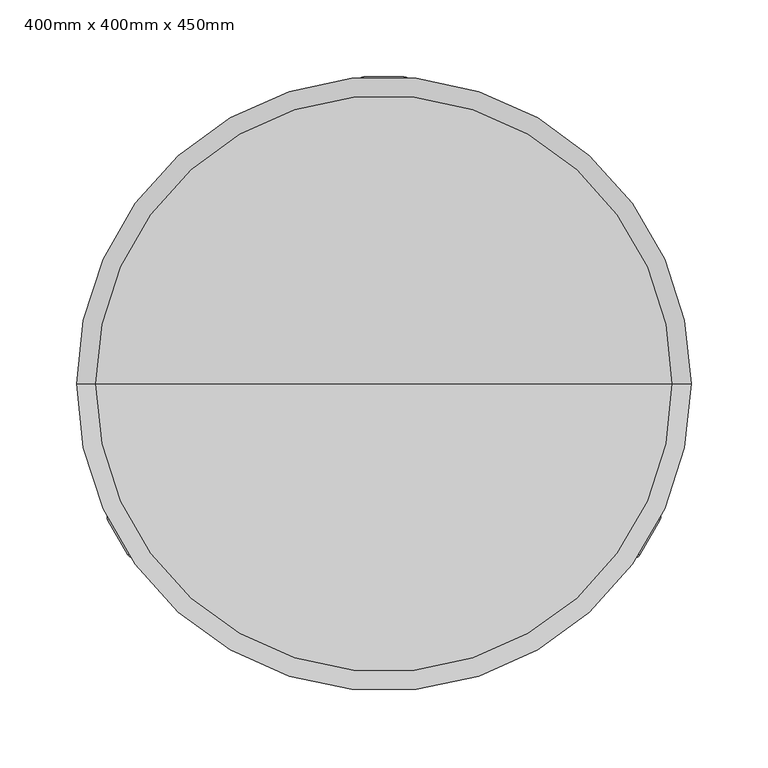
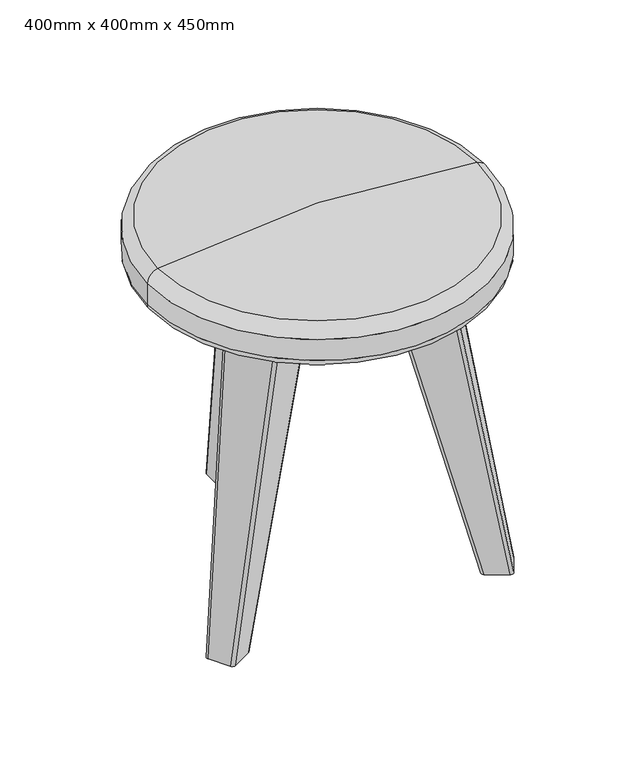
"""IFC4 building model written with IfcOpenShell, lengths in millimetres: furniture geometry, Seating-Casual-James_Burleigh-Shug : 400mm x 400mm x 450mm."""

from ifc_helpers import new_model, si_unit, point, frame, origin, place, context, project, spatial, circle_curve, ellipse_curve, trimmed, source, transform, mapped, element, save
from ifc_brep_helpers import plane_surface, cylinder_surface, revolved_surface, extruded_surface, advanced_brep


def furniture_400mm_x_400mm_x_450mm_e073d23b(model_context):
    return source(origin(), model_context, "Body", "AdvancedBrep", [
        advanced_brep(
        [(-100.6813787, -91.6147367, 384.0), (-95.2172771, -93.0788383, 384.0), (-44.9878037, -64.0788383, 384.0), (-43.5237021, -58.6147367, 384.0), (-72.5237021, -8.3852633, 384.0), (-77.9878037, -6.9211617, 384.0), (-128.2172771, -35.9211617, 384.0), (-129.6813787, -41.3852633, 384.0), (-166.7050808, -111.2583302, 0.0), (-179.7050808, -88.7416698, 0.0), (-178.2409791, -83.2775681, 0.0), (-155.7243186, -70.2775681, 0.0), (-150.260217, -71.7416698, 0.0), (-137.260217, -94.2583302, 0.0), (-138.7243186, -99.7224319, 0.0), (-161.2409791, -112.7224319, 0.0)],
        [
            (0, 1, circle_curve(frame((-97.2172771, -89.6147367, 384.0), z_axis=(0.0, 0.0, 1.0), x_axis=(-0.49999999999999306, 0.8660254037844427, 0.0)), 4.0)),
            (1, 2),
            (2, 3, circle_curve(frame((-46.9878037, -60.6147367, 384.0), z_axis=(0.0, 0.0, 1.0), x_axis=(-0.49999999999999306, 0.8660254037844427, 0.0)), 4.0)),
            (3, 4),
            (4, 5, circle_curve(frame((-75.9878037, -10.3852633, 384.0), z_axis=(0.0, 0.0, 1.0), x_axis=(-0.49999999999999306, 0.8660254037844427, 0.0)), 4.0)),
            (5, 6),
            (6, 7, circle_curve(frame((-126.2172771, -39.3852633, 384.0), z_axis=(0.0, 0.0, 1.0), x_axis=(-0.49999999999999306, 0.8660254037844427, 0.0)), 4.0)),
            (7, 0),
            (8, 9),
            (9, 10, circle_curve(frame((-176.2409791, -86.7416698, 0.0), z_axis=(0.0, 0.0, -1.0), x_axis=(-0.49999999999999306, 0.8660254037844427, 0.0)), 4.0)),
            (10, 11),
            (11, 12, circle_curve(frame((-153.7243186, -73.7416698, 0.0), z_axis=(0.0, 0.0, -1.0), x_axis=(-0.49999999999999306, 0.8660254037844427, 0.0)), 4.0)),
            (12, 13),
            (13, 14, circle_curve(frame((-140.7243186, -96.2583302, 0.0), z_axis=(0.0, 0.0, -1.0), x_axis=(-0.49999999999999306, 0.8660254037844427, 0.0)), 4.0)),
            (14, 15),
            (15, 8, circle_curve(frame((-163.2409791, -109.2583302, 0.0), z_axis=(0.0, 0.0, -1.0), x_axis=(-0.49999999999999306, 0.8660254037844427, 0.0)), 4.0)),
            (14, 2),
            (1, 15),
            (12, 4),
            (3, 13),
            (10, 6),
            (5, 11),
            (8, 0),
            (7, 9),
        ],
        [
            plane_surface(frame((-86.6025404, -50.0, 384.0), z_axis=(0.0, 0.0, 1.0), x_axis=(0.4999999999999859, -0.8660254037844468, 0.0))),
            plane_surface(frame((-158.4826489, -91.5, 0.0), z_axis=(0.0, 0.0, -1.0), x_axis=(0.4999999999999859, -0.8660254037844468, 0.0))),
            plane_surface(frame((-149.9826489, -106.2224319, 0.0), z_axis=(0.49956653654616645, -0.8652746230591969, -0.041630544712180834), x_axis=(0.8660254037844443, 0.4999999999999904, 0.0))),
            plane_surface(frame((-143.760217, -83.0, 0.0), z_axis=(0.8386038712126963, 0.4841681707881, -0.24964921306261928), x_axis=(-0.4999999999999904, 0.8660254037844443, 0.0))),
            plane_surface(frame((-166.9826489, -76.7775681, 0.0), z_axis=(-0.49956653654616634, 0.8652746230591967, -0.04163054471218183), x_axis=(-0.8660254037844443, -0.4999999999999904, 0.0))),
            plane_surface(frame((-173.2050808, -100.0, 0.0), z_axis=(-0.8531367483367913, -0.49255873130779587, 0.17188247394595313), x_axis=(0.4999999999999904, -0.8660254037844443, 0.0))),
            extruded_surface(trimmed(circle_curve(frame((-163.2409791, -109.2583302, 0.0), z_axis=(0.0, 0.0, 1.0), x_axis=(-0.49999999999999306, 0.8660254037844427, 0.0)), 4.0), [point((-166.7050808, -111.2583302, 0.0))], [point((-161.2409791, -112.7224319, 0.0))], True, "CARTESIAN"), (66.023702, 19.64359350000001, 384.0), 390.1294656795075),
            extruded_surface(trimmed(circle_curve(frame((-140.7243186, -96.2583302, 0.0), z_axis=(0.0, 0.0, 1.0), x_axis=(-0.49999999999999306, 0.8660254037844427, 0.0)), 4.0), [point((-138.7243186, -99.7224319, 0.0))], [point((-137.260217, -94.2583302, 0.0))], True, "CARTESIAN"), (93.7365149, 35.6435935, 384.0), 396.8790747610551),
            extruded_surface(trimmed(circle_curve(frame((-153.7243186, -73.7416698, 0.0), z_axis=(0.0, 0.0, 1.0), x_axis=(-0.49999999999999306, 0.8660254037844427, 0.0)), 4.0), [point((-150.260217, -71.7416698, 0.0))], [point((-155.7243186, -70.2775681, 0.0))], True, "CARTESIAN"), (77.7365149, 63.3564065, 384.0), 396.87907477390536),
            extruded_surface(trimmed(circle_curve(frame((-176.2409791, -86.7416698, 0.0), z_axis=(0.0, 0.0, 1.0), x_axis=(-0.49999999999999306, 0.8660254037844427, 0.0)), 4.0), [point((-178.2409791, -83.2775681, 0.0))], [point((-179.7050808, -88.7416698, 0.0))], True, "CARTESIAN"), (50.023702, 47.3564065, 384.0), 390.1294656884789),
        ],
        [
            (0, [[1, 2, 3, 4, 5, 6, 7, 8]]),
            (1, [[9, 10, 11, 12, 13, 14, 15, 16]]),
            (2, [[-15, 17, -2, 18]]),
            (3, [[-13, 19, -4, 20]]),
            (4, [[-11, 21, -6, 22]]),
            (5, [[-9, 23, -8, 24]]),
            (6, [[-16, -18, -1, -23]]),
            (7, [[-14, -20, -3, -17]]),
            (8, [[-12, -22, -5, -19]]),
            (9, [[-10, -24, -7, -21]]),
        ],
    ),
        advanced_brep(
        [(129.6813787, -41.3852633, 384.0), (128.2172771, -35.9211617, 384.0), (77.9878037, -6.9211617, 384.0), (72.5237021, -8.3852633, 384.0), (43.5237021, -58.6147367, 384.0), (44.9878037, -64.0788383, 384.0), (95.2172771, -93.0788383, 384.0), (100.6813787, -91.6147367, 384.0), (179.7050808, -88.7416698, 0.0), (166.7050808, -111.2583302, 0.0), (161.2409791, -112.7224319, 0.0), (138.7243186, -99.7224319, 0.0), (137.260217, -94.2583302, 0.0), (150.260217, -71.7416698, 0.0), (155.7243186, -70.2775681, 0.0), (178.2409791, -83.2775681, 0.0)],
        [
            (0, 1, circle_curve(frame((126.2172771, -39.3852633, 384.0), z_axis=(0.0, 0.0, 1.0000000000000002), x_axis=(-0.5000000000000088, -0.8660254037844337, 0.0)), 4.0)),
            (1, 2),
            (2, 3, circle_curve(frame((75.9878037, -10.3852633, 384.0), z_axis=(0.0, 0.0, 1.0000000000000002), x_axis=(-0.5000000000000088, -0.8660254037844337, 0.0)), 4.0)),
            (3, 4),
            (4, 5, circle_curve(frame((46.9878037, -60.6147367, 384.0), z_axis=(0.0, 0.0, 1.0000000000000002), x_axis=(-0.5000000000000088, -0.8660254037844337, 0.0)), 4.0)),
            (5, 6),
            (6, 7, circle_curve(frame((97.2172771, -89.6147367, 384.0), z_axis=(0.0, 0.0, 1.0000000000000002), x_axis=(-0.5000000000000088, -0.8660254037844337, 0.0)), 4.0)),
            (7, 0),
            (8, 9),
            (9, 10, circle_curve(frame((163.2409791, -109.2583302, 0.0), z_axis=(0.0, 0.0, -1.0000000000000002), x_axis=(-0.5000000000000088, -0.8660254037844337, 0.0)), 4.0)),
            (10, 11),
            (11, 12, circle_curve(frame((140.7243186, -96.2583302, 0.0), z_axis=(0.0, 0.0, -1.0000000000000002), x_axis=(-0.5000000000000088, -0.8660254037844337, 0.0)), 4.0)),
            (12, 13),
            (13, 14, circle_curve(frame((153.7243186, -73.7416698, 0.0), z_axis=(0.0, 0.0, -1.0000000000000002), x_axis=(-0.5000000000000088, -0.8660254037844337, 0.0)), 4.0)),
            (14, 15),
            (15, 8, circle_curve(frame((176.2409791, -86.7416698, 0.0), z_axis=(0.0, 0.0, -1.0000000000000002), x_axis=(-0.5000000000000088, -0.8660254037844337, 0.0)), 4.0)),
            (14, 2),
            (1, 15),
            (12, 4),
            (3, 13),
            (10, 6),
            (5, 11),
            (8, 0),
            (7, 9),
        ],
        [
            plane_surface(frame((86.6025404, -50.0, 384.0), z_axis=(0.0, 0.0, 1.0), x_axis=(0.5000000000000152, 0.8660254037844299, 0.0))),
            plane_surface(frame((158.4826489, -91.5, 0.0), z_axis=(0.0, 0.0, -1.0), x_axis=(0.5000000000000152, 0.8660254037844299, 0.0))),
            plane_surface(frame((166.9826489, -76.7775681, 0.0), z_axis=(0.49956653654618743, 0.8652746230591847, -0.041630544712180834), x_axis=(-0.8660254037844322, 0.5000000000000114, 0.0))),
            plane_surface(frame((143.760217, -83.0, 0.0), z_axis=(-0.8386038712126845, 0.48416817078812036, -0.24964921306261922), x_axis=(-0.5000000000000114, -0.8660254037844322, 0.0))),
            plane_surface(frame((149.9826489, -106.2224319, 0.0), z_axis=(-0.4995665365461874, -0.8652746230591846, -0.04163054471218185), x_axis=(0.8660254037844322, -0.5000000000000114, 0.0))),
            plane_surface(frame((173.2050808, -100.0, 0.0), z_axis=(0.8531367483367793, -0.4925587313078165, 0.17188247394595313), x_axis=(0.5000000000000114, 0.8660254037844322, 0.0))),
            extruded_surface(trimmed(circle_curve(frame((176.2409791, -86.7416698, 0.0), z_axis=(0.0, 0.0, 1.0000000000000002), x_axis=(-0.5000000000000088, -0.8660254037844337, 0.0)), 4.0), [point((179.7050808, -88.7416698, 0.0))], [point((178.2409791, -83.2775681, 0.0))], True, "CARTESIAN"), (-50.023702, 47.3564065, 384.0), 390.1294656884789),
            extruded_surface(trimmed(circle_curve(frame((153.7243186, -73.7416698, 0.0), z_axis=(0.0, 0.0, 1.0000000000000002), x_axis=(-0.5000000000000088, -0.8660254037844337, 0.0)), 4.0), [point((155.7243186, -70.2775681, 0.0))], [point((150.260217, -71.7416698, 0.0))], True, "CARTESIAN"), (-77.7365149, 63.3564065, 384.0), 396.87907477390536),
            extruded_surface(trimmed(circle_curve(frame((140.7243186, -96.2583302, 0.0), z_axis=(0.0, 0.0, 1.0000000000000002), x_axis=(-0.5000000000000088, -0.8660254037844337, 0.0)), 4.0), [point((137.260217, -94.2583302, 0.0))], [point((138.7243186, -99.7224319, 0.0))], True, "CARTESIAN"), (-93.7365149, 35.6435935, 384.0), 396.8790747610551),
            extruded_surface(trimmed(circle_curve(frame((163.2409791, -109.2583302, 0.0), z_axis=(0.0, 0.0, 1.0000000000000002), x_axis=(-0.5000000000000088, -0.8660254037844337, 0.0)), 4.0), [point((161.2409791, -112.7224319, 0.0))], [point((166.7050808, -111.2583302, 0.0))], True, "CARTESIAN"), (-66.023702, 19.64359350000001, 384.0), 390.1294656795075),
        ],
        [
            (0, [[1, 2, 3, 4, 5, 6, 7, 8]]),
            (1, [[9, 10, 11, 12, 13, 14, 15, 16]]),
            (2, [[-15, 17, -2, 18]]),
            (3, [[-13, 19, -4, 20]]),
            (4, [[-11, 21, -6, 22]]),
            (5, [[-9, 23, -8, 24]]),
            (6, [[-16, -18, -1, -23]]),
            (7, [[-14, -20, -3, -17]]),
            (8, [[-12, -22, -5, -19]]),
            (9, [[-10, -24, -7, -21]]),
        ],
    ),
        advanced_brep(
        [(-29.0, 133.0, 384.0), (-33.0, 129.0, 384.0), (-33.0, 71.0, 384.0), (-29.0, 67.0, 384.0), (29.0, 67.0, 384.0), (33.0, 71.0, 384.0), (33.0, 129.0, 384.0), (29.0, 133.0, 384.0), (-13.0, 200.0, 0.0), (13.0, 200.0, 0.0), (17.0, 196.0, 0.0), (17.0, 170.0, 0.0), (13.0, 166.0, 0.0), (-13.0, 166.0, 0.0), (-17.0, 170.0, 0.0), (-17.0, 196.0, 0.0)],
        [
            (0, 1, circle_curve(frame((-29.0, 129.0, 384.0), z_axis=(0.0, 0.0, 1.0), x_axis=(1.0, 0.0, 0.0)), 4.0)),
            (1, 2),
            (2, 3, circle_curve(frame((-29.0, 71.0, 384.0), z_axis=(0.0, 0.0, 1.0), x_axis=(1.0, 0.0, 0.0)), 4.0)),
            (3, 4),
            (4, 5, circle_curve(frame((29.0, 71.0, 384.0), z_axis=(0.0, 0.0, 1.0), x_axis=(1.0, 0.0, 0.0)), 4.0)),
            (5, 6),
            (6, 7, circle_curve(frame((29.0, 129.0, 384.0), z_axis=(0.0, 0.0, 1.0), x_axis=(1.0, 0.0, 0.0)), 4.0)),
            (7, 0),
            (8, 9),
            (9, 10, circle_curve(frame((13.0, 196.0, 0.0), z_axis=(0.0, 0.0, -1.0), x_axis=(1.0, 0.0, 0.0)), 4.0)),
            (10, 11),
            (11, 12, circle_curve(frame((13.0, 170.0, 0.0), z_axis=(0.0, 0.0, -1.0), x_axis=(1.0, 0.0, 0.0)), 4.0)),
            (12, 13),
            (13, 14, circle_curve(frame((-13.0, 170.0, 0.0), z_axis=(0.0, 0.0, -1.0), x_axis=(1.0, 0.0, 0.0)), 4.0)),
            (14, 15),
            (15, 8, circle_curve(frame((-13.0, 196.0, 0.0), z_axis=(0.0, 0.0, -1.0), x_axis=(1.0, 0.0, 0.0)), 4.0)),
            (14, 2),
            (1, 15),
            (12, 4),
            (3, 13),
            (10, 6),
            (5, 11),
            (8, 0),
            (7, 9),
        ],
        [
            plane_surface(frame((0.0, 100.0, 384.0), z_axis=(0.0, 0.0, 1.0), x_axis=(-1.0, 0.0, 0.0))),
            plane_surface(frame((0.0, 183.0, 0.0), z_axis=(0.0, 0.0, -1.0), x_axis=(-1.0, 0.0, 0.0))),
            plane_surface(frame((-17.0, 183.0, 0.0), z_axis=(-0.999133073092352, 0.0, -0.04163054471218082), x_axis=(0.0, -1.0, 0.0))),
            plane_surface(frame((0.0, 166.0, 0.0), z_axis=(0.0, -0.9683363415762186, -0.24964921306261917), x_axis=(1.0, 0.0, 0.0))),
            plane_surface(frame((17.0, 183.0, 0.0), z_axis=(0.999133073092352, 0.0, -0.04163054471218183), x_axis=(0.0, 1.0, 0.0))),
            plane_surface(frame((0.0, 200.0, 0.0), z_axis=(0.0, 0.9851174626156105, 0.1718824739459531), x_axis=(-1.0, 0.0, 0.0))),
            extruded_surface(trimmed(circle_curve(frame((-13.0, 196.0, 0.0), z_axis=(0.0, 0.0, 1.0), x_axis=(1.0, 0.0, 0.0)), 4.0), [point((-13.0, 200.0, 0.0))], [point((-17.0, 196.0, 0.0))], True, "CARTESIAN"), (-16.0, -67.0, 384.0), 390.12946569055765),
            extruded_surface(trimmed(circle_curve(frame((-13.0, 170.0, 0.0), z_axis=(0.0, 0.0, 1.0), x_axis=(1.0, 0.0, 0.0)), 4.0), [point((-17.0, 170.0, 0.0))], [point((-13.0, 166.0, 0.0))], True, "CARTESIAN"), (-16.0, -99.0, 384.0), 396.8790747822314),
            extruded_surface(trimmed(circle_curve(frame((13.0, 170.0, 0.0), z_axis=(0.0, 0.0, 1.0), x_axis=(1.0, 0.0, 0.0)), 4.0), [point((13.0, 166.0, 0.0))], [point((17.0, 170.0, 0.0))], True, "CARTESIAN"), (16.0, -99.0, 384.0), 396.8790747822314),
            extruded_surface(trimmed(circle_curve(frame((13.0, 196.0, 0.0), z_axis=(0.0, 0.0, 1.0), x_axis=(1.0, 0.0, 0.0)), 4.0), [point((17.0, 196.0, 0.0))], [point((13.0, 200.0, 0.0))], True, "CARTESIAN"), (16.0, -67.0, 384.0), 390.12946569055765),
        ],
        [
            (0, [[1, 2, 3, 4, 5, 6, 7, 8]]),
            (1, [[9, 10, 11, 12, 13, 14, 15, 16]]),
            (2, [[-15, 17, -2, 18]]),
            (3, [[-13, 19, -4, 20]]),
            (4, [[-11, 21, -6, 22]]),
            (5, [[-9, 23, -8, 24]]),
            (6, [[-16, -18, -1, -23]]),
            (7, [[-14, -20, -3, -17]]),
            (8, [[-12, -22, -5, -19]]),
            (9, [[-10, -24, -7, -21]]),
        ],
    ),
        advanced_brep(
        [(187.558801, 0.0, 434.7313492), (-187.558801, 0.0, 434.7313492), (0.0, 0.0, 450.0), (200.0, 0.0, 419.9512092), (-200.0, 0.0, 419.9512092), (200.0, 0.0, 394.0), (-200.0, 0.0, 394.0), (190.0, 0.0, 384.0), (-190.0, 0.0, 384.0), (0.0, 0.0, 384.0)],
        [
            (0, 1, circle_curve(frame((0.0, 0.0, 434.7313492), z_axis=(0.0, 0.0, 1.0), x_axis=(-1.0, 0.0, 0.0)), 187.558801)),
            (1, 2, circle_curve(frame((-9.3684334, 0.0, -594.5314254), z_axis=(0.0, 1.0, 0.0), x_axis=(1.0, 0.0, 0.0)), 1044.5734375)),
            (2, 0, circle_curve(frame((9.3684334, 0.0, -594.5314254), z_axis=(0.0, 1.0, 0.0), x_axis=(-1.0, 0.0, 0.0)), 1044.5734375)),
            (1, 0, circle_curve(frame((0.0, 0.0, 434.7313492), z_axis=(0.0, 0.0, 1.0), x_axis=(-1.0, 0.0, 0.0)), 187.558801)),
            (3, 4, circle_curve(frame((0.0, 0.0, 419.9512092), z_axis=(0.0, 0.0, 1.0), x_axis=(-1.0, 0.0, 0.0)), 200.0)),
            (4, 1, circle_curve(frame((-185.0, 0.0, 419.9512092), z_axis=(0.0, 1.0, 0.0), x_axis=(1.0, 0.0, 0.0)), 15.0)),
            (0, 3, circle_curve(frame((185.0, 0.0, 419.9512092), z_axis=(0.0, 1.0, 0.0), x_axis=(-1.0, 0.0, 0.0)), 15.0)),
            (4, 3, circle_curve(frame((0.0, 0.0, 419.9512092), z_axis=(0.0, 0.0, 1.0), x_axis=(-1.0, 0.0, 0.0)), 200.0)),
            (5, 6, circle_curve(frame((0.0, 0.0, 394.0), z_axis=(0.0, 0.0, 1.0), x_axis=(-1.0, 0.0, 0.0)), 200.0)),
            (6, 4),
            (3, 5),
            (6, 5, circle_curve(frame((0.0, 0.0, 394.0), z_axis=(0.0, 0.0, 1.0), x_axis=(-1.0, 0.0, 0.0)), 200.0)),
            (7, 8, circle_curve(frame((0.0, 0.0, 384.0), z_axis=(0.0, 0.0, 1.0), x_axis=(-1.0, 0.0, 0.0)), 190.0)),
            (8, 6, circle_curve(frame((-190.0, 0.0, 394.0), z_axis=(0.0, 1.0, 0.0), x_axis=(1.0, 0.0, 0.0)), 10.0)),
            (5, 7, circle_curve(frame((190.0, 0.0, 394.0), z_axis=(0.0, 1.0, 0.0), x_axis=(-1.0, 0.0, 0.0)), 10.0)),
            (8, 7, circle_curve(frame((0.0, 0.0, 384.0), z_axis=(0.0, 0.0, 1.0), x_axis=(-1.0, 0.0, 0.0)), 190.0)),
            (9, 8),
            (7, 9),
        ],
        [
            revolved_surface(trimmed(ellipse_curve(frame((-9.3684334, 0.0, -594.5314254), z_axis=(0.0, -1.0, 0.0), x_axis=(1.0, 0.0, 0.0)), 1044.5734375, 1044.5734375), [point((0.0, 0.0, 450.0))], [point((-187.558801, 0.0, 434.7313492))], True, "CARTESIAN"), (0.0, 0.0, 464.0), (0.0, 0.0, -1.0)),
            revolved_surface(trimmed(ellipse_curve(frame((-185.0, 0.0, 419.9512092), z_axis=(0.0, -1.0, 0.0), x_axis=(1.0, 0.0, 0.0)), 15.0, 15.0), [point((-187.558801, 0.0, 434.7313492))], [point((-200.0, 0.0, 419.9512092))], True, "CARTESIAN"), (0.0, 0.0, 464.0), (0.0, 0.0, -1.0)),
            cylinder_surface(frame((0.0, 0.0, 464.0), z_axis=(0.0, 0.0, -1.0), x_axis=(-1.0, 0.0, 0.0)), 200.0),
            revolved_surface(trimmed(ellipse_curve(frame((-190.0, 0.0, 394.0), z_axis=(0.0, -1.0, 0.0), x_axis=(1.0, 0.0, 0.0)), 10.0, 10.0), [point((-200.0, 0.0, 394.0))], [point((-190.0, 0.0, 384.0))], True, "CARTESIAN"), (0.0, 0.0, 464.0), (0.0, 0.0, -1.0)),
            plane_surface(frame((0.0, 0.0, 384.0), z_axis=(0.0, 0.0, -1.0), x_axis=(-1.0, 0.0, 0.0))),
        ],
        [
            (0, [[1, 2, 3]]),
            (0, [[4, -3, -2]]),
            (1, [[5, 6, -1, 7]]),
            (1, [[8, -7, -4, -6]]),
            (2, [[9, 10, -5, 11]]),
            (2, [[12, -11, -8, -10]]),
            (3, [[13, 14, -9, 15]]),
            (3, [[16, -15, -12, -14]]),
            (4, [[17, -13, 18]]),
            (4, [[-18, -16, -17]]),
        ],
    ),
    ])


if __name__ == "__main__":
    model = new_model("IFC4")
    model_context = context("Model", 3, world=origin())
    ifc_project = project(units=[si_unit("LENGTHUNIT", "METRE", prefix="MILLI")], contexts=[model_context])
    site = spatial("IfcSite", under=ifc_project)
    building = spatial("IfcBuilding", under=site)
    placement = place(None, origin())
    furniture_400mm_x_400mm_x_450mm_shape = furniture_400mm_x_400mm_x_450mm_e073d23b(model_context)
    element("IfcFurniture", 1, ObjectType="Seating-Casual-James_Burleigh-Shug : 400mm x 400mm x 450mm", at=placement, inside=building, context=model_context, shape_type="MappedRepresentation", body=[
        mapped(furniture_400mm_x_400mm_x_450mm_shape, transform((0.0, 0.0, 0.0), x_axis=(1.0, 0.0, 0.0), y_axis=(0.0, 1.0, 0.0), z_axis=(0.0, 0.0, 1.0))),
    ])
    save(model, "model.ifc")

# Revit data of these elements
# Type "Seating-Casual-James_Burleigh-Shug : 400mm x 400mm x 450mm"
#   _distributed by = "www.bimbox.co.uk"
#   _created by = "www.bimbox.co.uk"
#   _author = "BIMBox"
#   WarrantyStartDate [instance default] = "User Defined"
#   WarrantyGuarantorParts = "info@jamesburleigh.co.uk"
#   WarrantyGuarantorLabor = "info@jamesburleigh.co.uk"
#   WarrantyDurationUnit = "Years"
#   WarrantyDurationParts = "5"
#   WarrantyDurationLabor = "5"
#   WarrantyDescription = "5 Year Warranty on parts and labor"
#   Version = "1"
#   Uniclass2015 = "40.50.12.85"
#   URL = "www.jamesburleigh.co.uk"
#   TypeName = "400mm x 400mm x 450mm, Shug Stool"
#   Type Comments = "400mm x 400mm x 450mm"
#   TagNumber = "n/a"
#   SustainabilityPerformance = "n/a"
#   SpareParts = "n/a"
#   Size = "400x400x450"
#   Shape = "Rectangular"
#   SerialNumber = "n/a"
#   Revision = "1"
#   ReplacementCost = "0.00"
#   ProductInformation = "http://www.jamesburleigh.co.uk/contemporary-furniture/shug/"
#   Product URL = "http://www.jamesburleigh.co.uk/contemporary-furniture/shug/"
#   Option = "n/a"
#   Name = "Seating-Casual-James_Burleigh-Shug_Stool"
#   NBSReference = "40.50.12.85"
#   NBSDescription = "n/a"
#   ModelReference = "Shug Stool"
#   ModelNumber = "Shug"
#   Model = "Shug"
#   Material = "Various"
#   Manufacturer = "James Burleigh"
#   Keynote = "40.50.12.85"
#   InstallationDate [instance default] = "User Defined"
#   Grade = "Compact Grade"
#   Finish = "Contract use fabrics with solid wood legs"
#   Features = "Suitable for use in commercial, hospitality and leisure and education environments."
#   ExpectedLife = "25"
#   DurationUnit = "Years"
#   Description = "Shug Stool"
#   CreatedOn = "2015.04.17"
#   CreatedBy = "James Burleigh"
#   ContactTelephoneNumber = "+44 (0)20 8965 3966"
#   ContactFaxNumber = "n/a"
#   ContactEmailAddress = "info@jamesburleigh.co.uk"
#   Constituents = "n/a"
#   Color [instance default] = ""
#   CodePerformance = "n/a"
#   Category = "40.50.12.85 : Stools"
#   COBieDescription = "Shug, a substantial stool of modest proportions. Cleverly designed with three-point suspension for stability, Shug offers a sturdy solution to the problem of mobile seating in collaborative spaces and is suitable for all environments."
#   BarCode = "n/a"
#   BIMObjectName = "Seating-Casual-James_Burleigh-Shug_Stool"
#   AssetType = "Movable"
#   AssetIdentifier = "Shug"
#   Assembly Code = "E2020200"
#   AdditionalSurfaceFinishes = "Over 100 colours and wood grains for the surface with a range of solid wood birch ply edges."
#   AccessibilityPerformance = "n/a"
#   NominalWidth = 1' - 3.74803"
#   NominalLength = 1' - 3.74803"
#   NominalHeight = 1' - 5.71654"
#   _BIMspec_GUID = 0
#   Mtrl_Seat [instance default] = James_Burleigh-Fabric-Camira_Blazer-Newcastle_CUZ1W
#   Mtrl_LegEdge2 [instance default] = James_Burleigh-Wood-Oak_Leg_Side2
#   Mtrl_LegEdge1 [instance default] = James_Burleigh-Wood-Oak_Leg_Side
#   Mtrl_EdgeLeg [instance default] = James_Burleigh-Wood-Oak_Edge
#   Cost = 0
# Element 1 (IfcFurniture, "Seating-Casual-James_Burleigh-Shug : 400mm x 400mm x 450mm")
#   Materials on its faces: "James_Burleigh-Wood-Oak_Edge", "James_Burleigh-Fabric-Camira_Blazer-Newcastle_CUZ1W", "James_Burleigh-Wood-Oak_Leg_Side2", "James_Burleigh-Wood-Oak_Leg_Side"
# Materials
#   "James_Burleigh-Fabric-Camira_Blazer-Newcastle_CUZ1W": class "Miscellaneous", colour RGB 255 255 255, transparency 0, Model = "Blazer Kingsmead CUZ67", Manufacturer = "Camira", Cost = 0
#   "James_Burleigh-Wood-Oak_Leg_Side2": class "Generic", colour RGB 120 97 78, transparency 0, Cost = 0
#   "James_Burleigh-Wood-Oak_Leg_Side": class "Generic", colour RGB 124 101 81, transparency 0, Cost = 0
#   "James_Burleigh-Wood-Oak_Edge": class "Generic", colour RGB 116 92 74, transparency 0, Cost = 0
